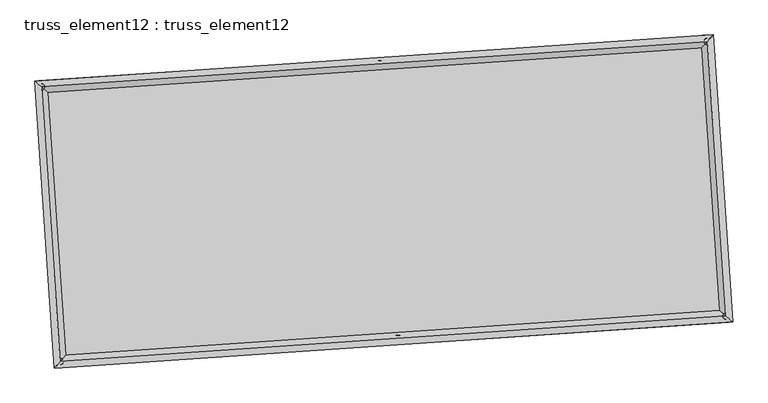
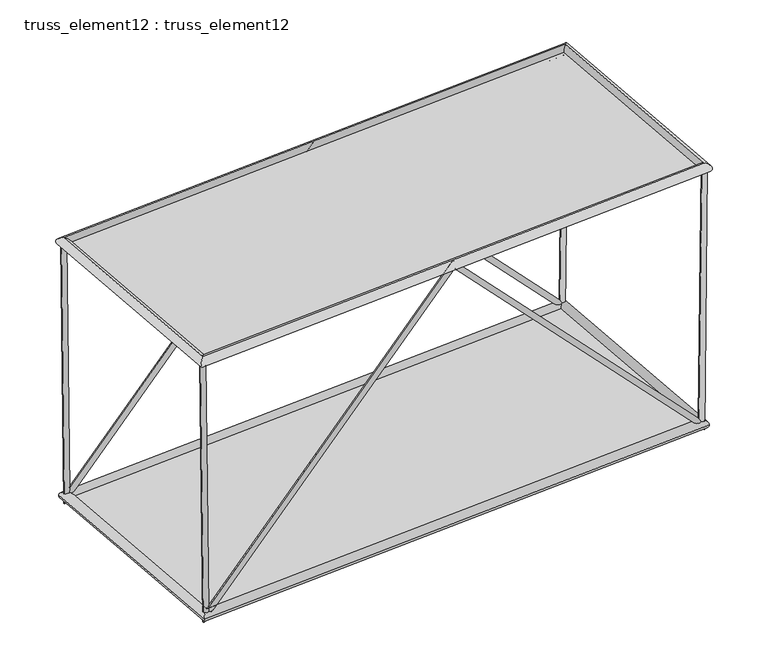
"""IFC4 building model written with IfcOpenShell, lengths in millimetres: plate geometry, truss_element12 : truss_element12."""

from ifc_helpers import new_model, si_unit, frame, origin, origin_with_axes, place, context, project, spatial, polyline, circle_curve, ellipse_curve, outline, extrude, source, transform, mapped, element, save
from ifc_brep_helpers import plane_surface, cylinder_surface, advanced_brep


def truss_element12_truss_element12_1e288aef(model_context):
    return source(origin(), model_context, "Body", "SolidModel", [
        advanced_brep(
        [(-3721.8541699, 2272.3433372, 5000.243792), (-3820.9510531, 2258.982503, 4999.1054445), (-3666.3357635, 2276.1289263, 122.7527544), (-3762.6511193, 2262.9577538, -122.7527544), (1063.2103796, 2598.6186991, 5071.8018953), (1063.6661844, 2592.0459842, 4927.5587941), (5793.7499875, 2921.1762125, 122.759853), (5891.0109895, 2921.204276, -122.759853), (5848.2824161, 2924.8945715, 5000.2451385), (5948.275935, 2925.108955, 4999.1270036)],
        [
            (0, 1, circle_curve(frame((-3771.4026115, 2265.6629201, 4999.6746183), z_axis=(-0.011381834017515616, -0.0007760839952527173, 0.9999349236565499), x_axis=(-0.13360848187270624, 0.9910339089151396, -0.0007516329220677924)), 50.0)),
            (1, 0, circle_curve(frame((-3771.4026115, 2265.6629201, 4999.6746183), z_axis=(-0.011381834017515616, -0.0007760839952527173, 0.9999349236565499), x_axis=(-0.13360848187270624, 0.9910339089151396, -0.0007516329220677924)), 50.0)),
            (0, 2),
            (2, 3, ellipse_curve(frame((-3714.4934414, 2269.54334, 0.0), z_axis=(-0.9278994784854547, -0.06326993816178475, 0.36742274392234436), x_axis=(0.36657157095159426, 0.024995121954192616, 0.9300540453374608)), 132.271936, 50.0)),
            (3, 1),
            (3, 2, ellipse_curve(frame((-3714.4934414, 2269.54334, 0.0), z_axis=(-0.9278994784854547, -0.06326993816178475, 0.36742274392234436), x_axis=(0.36657157095159426, 0.024995121954192616, 0.9300540453374608)), 132.271936, 50.0)),
            (2, 4),
            (4, 5, ellipse_curve(frame((1063.438282, 2595.3323417, 4999.6803447), z_axis=(-0.9976833946832313, -0.06802823813381093, -5.281811364997211e-05), x_axis=(5.2695755000598474e-05, 3.593123218122507e-06, -0.9999999986051235)), 72.2785958, 50.0)),
            (5, 3),
            (5, 4, ellipse_curve(frame((1063.438282, 2595.3323417, 4999.6803447), z_axis=(-0.9976833946832313, -0.06802823813381093, -5.281811364997211e-05), x_axis=(5.2695755000598474e-05, 3.593123218122507e-06, -0.9999999986051235)), 72.2785958, 50.0)),
            (4, 6),
            (6, 7, ellipse_curve(frame((5842.3804885, 2921.1902443, 0.0), z_axis=(-0.9278429760300568, -0.06326608547413708, -0.3675660678850353), x_axis=(-0.3667145628894308, -0.025004872030870366, 0.9299974116843194)), 132.2876405, 50.0)),
            (7, 5),
            (7, 6, ellipse_curve(frame((5842.3804885, 2921.1902443, 0.0), z_axis=(-0.9278429760300568, -0.06326608547413708, -0.3675660678850353), x_axis=(-0.3667145628894308, -0.025004872030870366, 0.9299974116843194)), 132.2876405, 50.0)),
            (8, 9, circle_curve(frame((5898.2791756, 2925.0017632, 4999.6860711), z_axis=(0.011179737411862272, 0.0007623037959543959, 0.9999372142111346), x_axis=(-0.002152223979418104, 0.9999974114288641, -0.0007382868776594081)), 50.0)),
            (9, 8, circle_curve(frame((5898.2791756, 2925.0017632, 4999.6860711), z_axis=(0.011179737411862272, 0.0007623037959543959, 0.9999372142111346), x_axis=(-0.002152223979418104, 0.9999974114288641, -0.0007382868776594081)), 50.0)),
            (6, 8),
            (9, 7),
        ],
        [
            plane_surface(frame((-3771.4026115, 2315.662905, 4999.713425), z_axis=(-0.01138183401751662, -0.0007760839952526837, 0.99993492365655), x_axis=(0.9999352248292876, -8.833831430798961e-06, 0.01138183058939645))),
            cylinder_surface(frame((-3771.4026115, 2265.6629201, 4999.6746183), z_axis=(-0.011381834017515616, -0.0007760839952527173, 0.9999349236565499), x_axis=(-0.13360848187270624, 0.9910339089151396, -0.0007516329220677924)), 50.0),
            cylinder_surface(frame((-3714.4934414, 2269.54334, 0.0), z_axis=(-0.6901271226391988, -0.04705714507397151, -0.7221566171511742), x_axis=(-0.0204113902098155, 0.9987523882932022, -0.045574576556754245)), 50.0),
            cylinder_surface(frame((1063.438282, 2595.3323417, 4999.6803447), z_axis=(-0.690203227964863, -0.04706233440682505, 0.72208354141821), x_axis=(-0.11534466276751382, 0.9922792493126465, -0.04557960239601923)), 50.0),
            plane_surface(frame((5898.2791756, 2875.0017778, 4999.7241886), z_axis=(0.011179737411861788, 0.0007623037959489832, 0.9999372142111346), x_axis=(0.9999375047828748, -8.522888906625786e-06, -0.011179734163143003))),
            cylinder_surface(frame((5842.3804885, 2921.1902443, 0.0), z_axis=(-0.011179737411862274, -0.0007623037959543961, -0.9999372142111348), x_axis=(-0.002152223979418104, 0.9999974114288641, -0.0007382868776594081)), 50.0),
        ],
        [
            (0, [[1, 2]]),
            (1, [[-1, 3, 4, 5]]),
            (1, [[-2, -5, 6, -3]]),
            (2, [[-4, 7, 8, 9]]),
            (2, [[-6, -9, 10, -7]]),
            (3, [[-8, 11, 12, 13]]),
            (3, [[-10, -13, 14, -11]]),
            (4, [[15, 16]]),
            (5, [[-12, 17, -16, 18]]),
            (5, [[-14, -18, -15, -17]]),
        ],
    ),
        advanced_brep(
        [(-3449.741217, -1718.3902471, 5000.243792), (-3548.8381002, -1731.7510813, 4999.1054445), (-3394.2228106, -1714.604658, 122.7527544), (-3490.5381664, -1727.7758305, -122.7527544), (1335.3233326, -1392.1148852, 5071.8018953), (1335.7791373, -1398.6876001, 4927.5587941), (6065.8629405, -1069.5573718, 122.759853), (6163.1239424, -1069.5293083, -122.759853), (6120.395369, -1065.8390128, 5000.2451385), (6220.3888879, -1065.6246293, 4999.1270036)],
        [
            (0, 1, circle_curve(frame((-3499.2896586, -1725.0706642, 4999.6746183), z_axis=(-0.0113818340175155, -0.0007760839952527034, 0.9999349236565499), x_axis=(-0.1336084818727064, 0.9910339089151396, -0.0007516329220677924)), 50.0)),
            (1, 0, circle_curve(frame((-3499.2896586, -1725.0706642, 4999.6746183), z_axis=(-0.0113818340175155, -0.0007760839952527034, 0.9999349236565499), x_axis=(-0.1336084818727064, 0.9910339089151396, -0.0007516329220677924)), 50.0)),
            (0, 2),
            (2, 3, ellipse_curve(frame((-3442.3804885, -1721.1902443, 0.0), z_axis=(-0.927899478485455, -0.06326993816178478, 0.3674227439223443), x_axis=(0.36657157095159415, 0.02499512195419262, 0.9300540453374606)), 132.271936, 50.0)),
            (3, 1),
            (3, 2, ellipse_curve(frame((-3442.3804885, -1721.1902443, 0.0), z_axis=(-0.927899478485455, -0.06326993816178478, 0.3674227439223443), x_axis=(0.36657157095159415, 0.02499512195419262, 0.9300540453374606)), 132.271936, 50.0)),
            (2, 4),
            (4, 5, ellipse_curve(frame((1335.5512349, -1395.4012426, 4999.6803447), z_axis=(-0.9976833946832313, -0.06802823813381102, -5.281811365021285e-05), x_axis=(5.269575500075221e-05, 3.59312321818977e-06, -0.9999999986051235)), 72.2785958, 50.0)),
            (5, 3),
            (5, 4, ellipse_curve(frame((1335.5512349, -1395.4012426, 4999.6803447), z_axis=(-0.9976833946832313, -0.06802823813381102, -5.281811365021285e-05), x_axis=(5.269575500075221e-05, 3.59312321818977e-06, -0.9999999986051235)), 72.2785958, 50.0)),
            (4, 6),
            (6, 7, ellipse_curve(frame((6114.4934414, -1069.54334, 0.0), z_axis=(-0.9278429760300566, -0.06326608547413719, -0.36756606788503576), x_axis=(-0.3667145628894313, -0.025004872030870456, 0.9299974116843193)), 132.2876405, 50.0)),
            (7, 5),
            (7, 6, ellipse_curve(frame((6114.4934414, -1069.54334, 0.0), z_axis=(-0.9278429760300566, -0.06326608547413719, -0.36756606788503576), x_axis=(-0.3667145628894313, -0.025004872030870456, 0.9299974116843193)), 132.2876405, 50.0)),
            (8, 9, circle_curve(frame((6170.3921285, -1065.7318211, 4999.6860711), z_axis=(0.011179737411862045, 0.0007623037959543686, 0.9999372142111348), x_axis=(-0.0021522239794181794, 0.999997411428864, -0.0007382868776593801)), 50.0)),
            (9, 8, circle_curve(frame((6170.3921285, -1065.7318211, 4999.6860711), z_axis=(0.011179737411862045, 0.0007623037959543686, 0.9999372142111348), x_axis=(-0.0021522239794181794, 0.999997411428864, -0.0007382868776593801)), 50.0)),
            (6, 8),
            (9, 7),
        ],
        [
            plane_surface(frame((-3499.2896586, -1675.0706793, 4999.713425), z_axis=(-0.01138183401751662, -0.0007760839952526816, 0.99993492365655), x_axis=(0.9999352248292876, -8.833831430798961e-06, 0.01138183058939645))),
            cylinder_surface(frame((-3499.2896586, -1725.0706642, 4999.6746183), z_axis=(-0.0113818340175155, -0.0007760839952527034, 0.9999349236565499), x_axis=(-0.1336084818727064, 0.9910339089151396, -0.0007516329220677924)), 50.0),
            cylinder_surface(frame((-3442.3804885, -1721.1902443, 0.0), z_axis=(-0.6901271226391986, -0.04705714507397152, -0.7221566171511744), x_axis=(-0.020411390209815434, 0.9987523882932022, -0.045574576556754315)), 50.0),
            cylinder_surface(frame((1335.5512349, -1395.4012426, 4999.6803447), z_axis=(-0.6902032279648631, -0.047062334406825154, 0.7220835414182099), x_axis=(-0.11534466276751408, 0.9922792493126465, -0.04557960239601936)), 50.0),
            plane_surface(frame((6170.3921285, -1115.7318065, 4999.7241886), z_axis=(0.011179737411861788, 0.0007623037959489812, 0.9999372142111346), x_axis=(0.9999375047828748, -8.522888906625786e-06, -0.011179734163143003))),
            cylinder_surface(frame((6114.4934414, -1069.54334, 0.0), z_axis=(-0.011179737411862043, -0.0007623037959543684, -0.9999372142111346), x_axis=(-0.0021522239794181794, 0.999997411428864, -0.0007382868776593801)), 50.0),
        ],
        [
            (0, [[1, 2]]),
            (1, [[-1, 3, 4, 5]]),
            (1, [[-2, -5, 6, -3]]),
            (2, [[-4, 7, 8, 9]]),
            (2, [[-6, -9, 10, -7]]),
            (3, [[-8, 11, 12, 13]]),
            (3, [[-10, -13, 14, -11]]),
            (4, [[15, 16]]),
            (5, [[-12, 17, -16, 18]]),
            (5, [[-14, -18, -15, -17]]),
        ],
    ),
        advanced_brep(
        [(-3499.2866492, -1725.0673288, 4909.6746183), (-3499.292668, -1725.0739997, 5089.6746182), (-3771.4060458, 2265.6658161, 5089.6746182), (-3771.3991772, 2265.660024, 4909.6746183), (5898.2819728, 2925.0050842, 5089.686071), (5898.2763784, 2924.9984423, 4909.6860711), (6170.3953506, -1065.7347316, 5089.686071), (6170.3889064, -1065.7289105, 4909.6860711)],
        [
            (0, 1, ellipse_curve(frame((-3499.2896586, -1725.0706642, 4999.6746183), z_axis=(-0.7535719234049658, 0.657365466278114, -8.3555725473804e-07), x_axis=(-0.6573654662775879, -0.7535719234054246, -8.355572547380254e-07)), 127.2792206, 90.0)),
            (1, 2),
            (2, 3, ellipse_curve(frame((-3771.4026115, 2265.6629201, 4999.6746183), z_axis=(-0.6573654662775877, -0.7535719234054249, -8.355572547380119e-07), x_axis=(0.7535719234049659, -0.6573654662781139, 8.355572547380267e-07)), 127.2792206, 90.0)),
            (3, 0),
            (1, 0, ellipse_curve(frame((-3499.2896586, -1725.0706642, 4999.6746183), z_axis=(-0.7535719234049658, 0.657365466278114, -8.3555725473804e-07), x_axis=(-0.6573654662775879, -0.7535719234054246, -8.355572547380254e-07)), 127.2792206, 90.0)),
            (3, 2, ellipse_curve(frame((-3771.4026115, 2265.6629201, 4999.6746183), z_axis=(-0.6573654662775877, -0.7535719234054249, -8.355572547380119e-07), x_axis=(0.7535719234049659, -0.6573654662781139, 8.355572547380267e-07)), 127.2792206, 90.0)),
            (2, 4),
            (4, 5, ellipse_curve(frame((5898.2791756, 2925.0017632, 4999.6860711), z_axis=(-0.7535719234049658, 0.657365466278114, -8.355572547380136e-07), x_axis=(-0.6573654662775879, -0.7535719234054248, -8.355572547380251e-07)), 127.2792206, 90.0)),
            (5, 3),
            (5, 4, ellipse_curve(frame((5898.2791756, 2925.0017632, 4999.6860711), z_axis=(-0.7535719234049658, 0.657365466278114, -8.355572547380136e-07), x_axis=(-0.6573654662775879, -0.7535719234054248, -8.355572547380251e-07)), 127.2792206, 90.0)),
            (4, 6),
            (6, 7, ellipse_curve(frame((6170.3921285, -1065.7318211, 4999.6860711), z_axis=(0.6573654662775877, 0.7535719234054248, 8.355572547380384e-07), x_axis=(-0.7535719234049659, 0.657365466278114, -8.355572547380273e-07)), 127.2792206, 90.0)),
            (7, 5),
            (7, 6, ellipse_curve(frame((6170.3921285, -1065.7318211, 4999.6860711), z_axis=(0.6573654662775877, 0.7535719234054248, 8.355572547380384e-07), x_axis=(-0.7535719234049659, 0.657365466278114, -8.355572547380273e-07)), 127.2792206, 90.0)),
            (6, 1),
            (0, 7),
        ],
        [
            cylinder_surface(frame((-3499.2896586, -1725.0706642, 4999.6746183), z_axis=(0.06802823822870131, -0.9976833960748765, 0.0), x_axis=(-0.9976833954326236, -0.06802823818490852, -3.58815903472379e-05)), 90.0),
            cylinder_surface(frame((-3771.4026115, 2265.6629201, 4999.6746183), z_axis=(-0.99768339607418, -0.06802823822865506, -1.1816564017897381e-06), x_axis=(-0.06802823814683823, 0.9976833954770179, -3.4699933946159566e-05)), 90.0),
            cylinder_surface(frame((5898.2791756, 2925.0017632, 4999.6860711), z_axis=(-0.06802823822870106, 0.9976833960748765, 0.0), x_axis=(0.9976833955144404, 0.06802823819048705, -3.351827754508122e-05)), 90.0),
            cylinder_surface(frame((6170.3921285, -1065.7318211, 4999.6860711), z_axis=(0.99768339607418, 0.06802823822865493, 1.181656401789757e-06), x_axis=(0.06802823822865493, -0.9976833954714391, -3.469993394615955e-05)), 90.0),
        ],
        [
            (0, [[1, 2, 3, 4]]),
            (0, [[5, -4, 6, -2]]),
            (1, [[-3, 7, 8, 9]]),
            (1, [[-6, -9, 10, -7]]),
            (2, [[-8, 11, 12, 13]]),
            (2, [[-10, -13, 14, -11]]),
            (3, [[-12, 15, -1, 16]]),
            (3, [[-14, -16, -5, -15]]),
        ],
    ),
        advanced_brep(
        [(-3358.7115243, -1625.2761972, 0.0), (-3526.0494527, -1817.1042913, 0.0), (-3810.4074885, 2353.2123043, 0.0), (-3618.5793943, 2185.8743758, 0.0), (5926.0494527, 3017.1042913, 0.0), (5758.7115243, 2825.2761972, 0.0), (6210.4074885, -1153.2123043, 0.0), (6018.5793943, -985.8743758, 0.0)],
        [
            (0, 1, ellipse_curve(frame((-3442.3804885, -1721.1902443, 0.0), z_axis=(-0.7535719234054579, 0.6573654662780809, 0.0), x_axis=(-0.657365466278081, -0.7535719234054578, 0.0)), 127.2792206, 90.0)),
            (1, 2),
            (2, 3, ellipse_curve(frame((-3714.4934414, 2269.54334, 0.0), z_axis=(-0.6573654662780808, -0.7535719234054579, 0.0), x_axis=(0.7535719234054578, -0.6573654662780809, 0.0)), 127.2792206, 90.0)),
            (3, 0),
            (1, 0, ellipse_curve(frame((-3442.3804885, -1721.1902443, 0.0), z_axis=(-0.7535719234054579, 0.6573654662780809, 0.0), x_axis=(-0.657365466278081, -0.7535719234054578, 0.0)), 127.2792206, 90.0)),
            (3, 2, ellipse_curve(frame((-3714.4934414, 2269.54334, 0.0), z_axis=(-0.6573654662780808, -0.7535719234054579, 0.0), x_axis=(0.7535719234054578, -0.6573654662780809, 0.0)), 127.2792206, 90.0)),
            (2, 4),
            (4, 5, ellipse_curve(frame((5842.3804885, 2921.1902443, 0.0), z_axis=(-0.7535719234054579, 0.6573654662780809, 0.0), x_axis=(-0.6573654662780809, -0.7535719234054578, 0.0)), 127.2792206, 90.0)),
            (5, 3),
            (5, 4, ellipse_curve(frame((5842.3804885, 2921.1902443, 0.0), z_axis=(-0.7535719234054579, 0.6573654662780809, 0.0), x_axis=(-0.6573654662780809, -0.7535719234054578, 0.0)), 127.2792206, 90.0)),
            (4, 6),
            (6, 7, ellipse_curve(frame((6114.4934414, -1069.54334, 0.0), z_axis=(0.6573654662780809, 0.7535719234054579, 0.0), x_axis=(-0.7535719234054578, 0.6573654662780809, 0.0)), 127.2792206, 90.0)),
            (7, 5),
            (7, 6, ellipse_curve(frame((6114.4934414, -1069.54334, 0.0), z_axis=(0.6573654662780809, 0.7535719234054579, 0.0), x_axis=(-0.7535719234054578, 0.6573654662780809, 0.0)), 127.2792206, 90.0)),
            (6, 1),
            (0, 7),
        ],
        [
            cylinder_surface(frame((-3442.3804885, -1721.1902443, 0.0), z_axis=(0.06802823822870059, -0.9976833960748767, 0.0), x_axis=(-0.9976833960748767, -0.06802823822870059, 0.0)), 90.0),
            cylinder_surface(frame((-3714.4934414, 2269.54334, 0.0), z_axis=(-0.9976833960748767, -0.06802823822870172, 0.0), x_axis=(-0.06802823822870172, 0.9976833960748767, 0.0)), 90.0),
            cylinder_surface(frame((5842.3804885, 2921.1902443, 0.0), z_axis=(-0.06802823822870048, 0.9976833960748768, 0.0), x_axis=(0.9976833960748768, 0.06802823822870048, 0.0)), 90.0),
            cylinder_surface(frame((6114.4934414, -1069.54334, 0.0), z_axis=(0.9976833960748767, 0.06802823822870152, 0.0), x_axis=(0.06802823822870152, -0.9976833960748767, 0.0)), 90.0),
        ],
        [
            (0, [[1, 2, 3, 4]]),
            (0, [[5, -4, 6, -2]]),
            (1, [[-3, 7, 8, 9]]),
            (1, [[-6, -9, 10, -7]]),
            (2, [[-8, 11, 12, 13]]),
            (2, [[-10, -13, 14, -11]]),
            (3, [[-12, 15, -1, 16]]),
            (3, [[-14, -16, -5, -15]]),
        ],
    ),
        extrude(outline(polyline([(-3442.3804885, -1721.1902443), (-3714.4934414, 2269.54334), (5842.3804885, 2921.1902443), (6114.4934414, -1069.54334), (-3442.3804885, -1721.1902443)])), origin_with_axes(), (0.0, 0.0, 1.0), 20.0),
        extrude(outline(polyline([(-2000.0, 4846.0673121), (2000.0, 4846.0673121), (2000.0, -4846.0673121), (-2000.0, -4846.0673121), (-2000.0, 4846.0673121)])), frame((1199.4947585, 599.9655495, 4999.6803447), z_axis=(-1.1789189719312138e-06, -8.038600320542223e-08, 0.9999999999993019), x_axis=(-0.06802823822870074, 0.9976833960748767, 0.0)), (0.0, 0.0, 1.0), 20.0),
    ])


if __name__ == "__main__":
    model = new_model("IFC4")
    model_context = context("Model", 3, world=origin())
    ifc_project = project(units=[si_unit("LENGTHUNIT", "METRE", prefix="MILLI")], contexts=[model_context])
    site = spatial("IfcSite", under=ifc_project)
    building = spatial("IfcBuilding", under=site)
    placement = place(None, origin())
    truss_element12_truss_element12_shape = truss_element12_truss_element12_1e288aef(model_context)
    element("IfcPlate", 1, ObjectType="truss_element12 : truss_element12", at=placement, inside=building, context=model_context, shape_type="MappedRepresentation", body=[
        mapped(truss_element12_truss_element12_shape, transform((0.0, 0.0, 0.0), x_axis=(1.0, 0.0, 0.0), y_axis=(0.0, 1.0, 0.0), z_axis=(0.0, 0.0, 1.0))),
    ])
    save(model, "model.ifc")

# Revit data of these elements
# Type "truss_element12 : truss_element12"
#   steellbar1 = 90 mm
#   steelbar2 = 50 mm
#   offset1 = 5000 mm
#   M = Default Roof
# Element 1 (IfcPlate, "truss_element12 : truss_element12")
#   Materials on its faces: "Default Roof"
# Materials
#   "Default Roof": class "Miscellaneous", colour RGB 0 127 0, transparency 0, Comments = "Rendering appearance not upgraded Rendering appearance not upgraded ", Cost = 0
